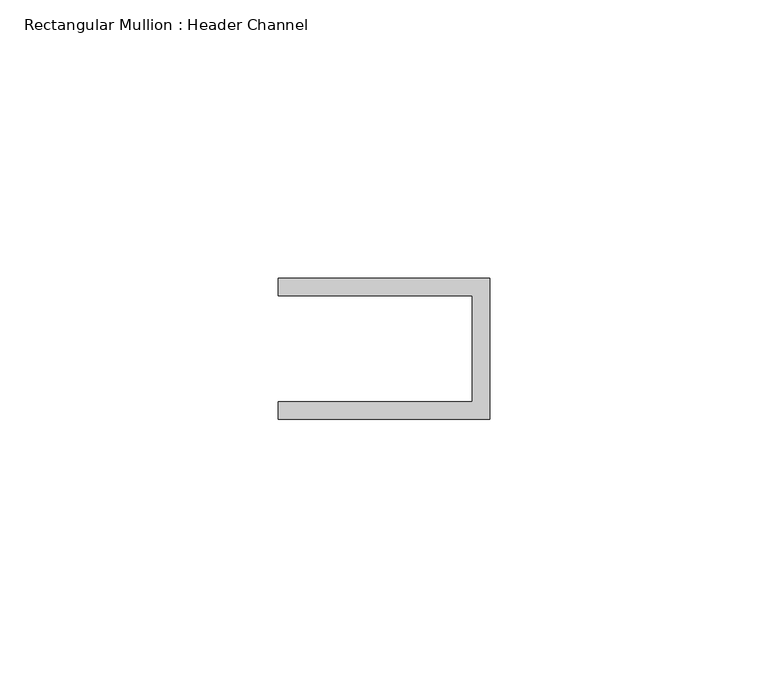
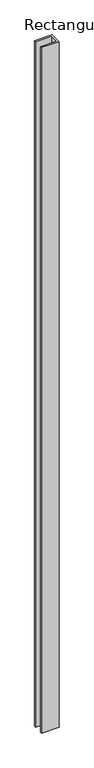
"""IFC4 building model written with IfcOpenShell, lengths in millimetres: member geometry, Rectangular Mullion : Header Channel."""

from ifc_helpers import new_model, si_unit, frame, origin, place, context, project, spatial, polyline, outline, extrude, source, transform, mapped, element, save


def rectangular_mullion_header_channel_792eb991(model_context):
    return source(origin(), model_context, "Body", "SweptSolid", [
        extrude(outline(polyline([(0.0, 12.7), (0.0, -12.7), (-38.1, -12.7), (-38.1, -9.525), (-3.175, -9.525), (-3.175, 9.525), (-38.1, 9.525), (-38.1, 12.7), (0.0, 12.7)])), frame((0.0, 0.0, -1581.15), z_axis=(0.0, 0.0, 1.0), x_axis=(1.0, 0.0, 0.0)), (0.0, 0.0, 1.0), 1581.15),
    ])


if __name__ == "__main__":
    model = new_model("IFC4")
    model_context = context("Model", 3, world=origin())
    ifc_project = project(units=[si_unit("LENGTHUNIT", "METRE", prefix="MILLI")], contexts=[model_context])
    site = spatial("IfcSite", under=ifc_project)
    building = spatial("IfcBuilding", under=site)
    placement = place(None, origin())
    rectangular_mullion_header_channel_shape = rectangular_mullion_header_channel_792eb991(model_context)
    element("IfcMember", 1, ObjectType="Rectangular Mullion : Header Channel", at=placement, inside=building, context=model_context, shape_type="MappedRepresentation", body=[
        mapped(rectangular_mullion_header_channel_shape, transform((0.0, 0.0, 0.0), x_axis=(1.0, 0.0, 0.0), y_axis=(0.0, 1.0, 0.0), z_axis=(0.0, 0.0, 1.0))),
    ])
    save(model, "model.ifc")

# Revit data of these elements
# Type "Rectangular Mullion : Header Channel"
#   built-in parameter 1007322 = 0.0833333 (stored number, unit not read)
#   built-in parameter 1007321 = -0.03125 (stored number, unit not read)
#   built-in parameter 1007320 = 0.0416667 (stored number, unit not read)
# Element 1 (IfcMember, "Rectangular Mullion : Header Channel")
#   Materials on its faces: "ALUM"
# Materials
#   "ALUM": class "Generic", colour RGB 157 157 157, transparency 0, Cost = 0
